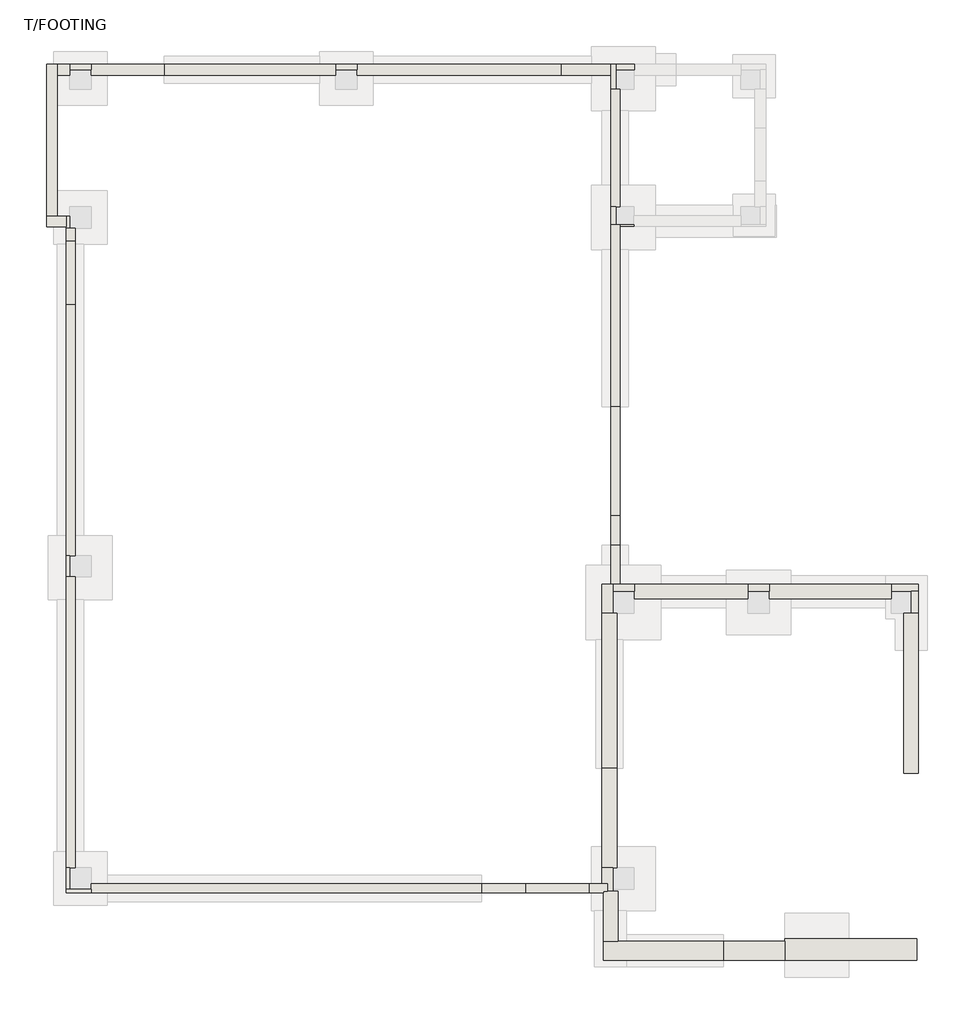
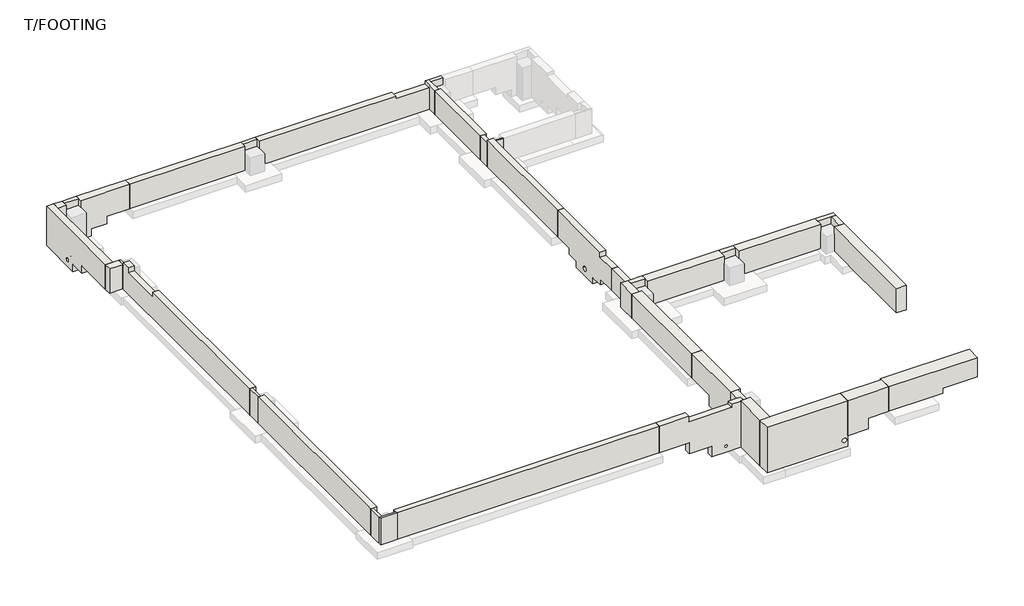
# One storey, part 1 of 3: 39 walls.
"""IFC4 building model written with IfcOpenShell, lengths in millimetres."""

from ifc_helpers import new_model, si_unit, point, frame, frame_2d, origin, place, context, project, spatial, polyline, circle_curve, trimmed, segment, composite_curve, outline, extrude, faceted_brep, element, save
from ifc_brep_helpers import plane_surface, revolved_surface, advanced_brep

model = new_model("IFC4")

# Units and contexts
model_context = context("Model", 3, world=origin())
ifc_project = project(units=[si_unit("LENGTHUNIT", "METRE", prefix="MILLI")], contexts=[model_context])

# Site, building, storey
site = spatial("IfcSite", under=ifc_project)
building = spatial("IfcBuilding", under=site)
storey = spatial("IfcBuildingStorey", under=building, Name="T/FOOTING", Elevation=-1092.2)

# Walls
placement = place(None, origin())
element("IfcWall", 1, ObjectType="10\" CONCRETE WALL", at=placement, inside=storey, context=model_context, shape_type="AdvancedBrep", body=[
    advanced_brep(
    [(-51687.4600821, -10190.4231529, -1092.2), (-52957.4600821, -10190.4231529, -1092.2), (-52957.4600821, -10190.4231529, 101.6), (-51700.1600824, -10190.4231529, 101.6), (-51700.1600824, -10190.4231529, -127.0), (-49871.3600824, -10190.4231529, -127.0), (-49871.3600824, -10190.4231529, 0.0), (-49512.5850821, -10190.4231529, 0.0), (-49360.1850821, -10190.4231529, 0.0), (-49360.1850821, -10190.4231529, -2057.4), (-49512.5850821, -10190.4231529, -2057.4), (-50722.2600821, -10190.4231529, -2057.4), (-50722.2600821, -10190.4231529, -1574.8), (-51687.4600821, -10190.4231529, -1574.8), (-50163.4600821, -10190.4231529, -1790.7), (-50061.8600821, -10190.4231529, -1790.7), (-52957.4600821, -10444.4231529, -1092.2), (-51687.4600821, -10444.4231529, -1092.2), (-51687.4600821, -10444.4231529, -1574.8), (-50722.2600821, -10444.4231529, -1574.8), (-50722.2600821, -10444.4231529, -2057.4), (-49477.6600821, -10444.4231529, -2057.4), (-49477.6600821, -10444.4231529, 0.0), (-49871.3600824, -10444.4231529, 0.0), (-49871.3600824, -10444.4231529, -127.0), (-51700.1600824, -10444.4231529, -127.0), (-51700.1600824, -10444.4231529, 101.6), (-52957.4600821, -10444.4231529, 101.6), (-50061.8600821, -10444.4231529, -1790.7), (-50163.4600821, -10444.4231529, -1790.7), (-49360.1850821, -10393.6231529, 0.0), (-49360.1850821, -10393.6231529, -2057.4), (-49477.6600821, -10393.6231529, -2057.4), (-49477.6600821, -10393.6231529, 0.0)],
    [
        (0, 1),
        (1, 2),
        (2, 3),
        (3, 4),
        (4, 5),
        (5, 6),
        (6, 7),
        (7, 8),
        (8, 9),
        (9, 10),
        (10, 11),
        (11, 12),
        (12, 13),
        (13, 0),
        (14, 15, circle_curve(frame((-50112.6600821, -10190.4231529, -1790.7), z_axis=(0.0, -1.0, 0.0), x_axis=(1.0, 0.0, 0.0)), 50.8)),
        (15, 14, circle_curve(frame((-50112.6600821, -10190.4231529, -1790.7), z_axis=(0.0, -1.0, 0.0), x_axis=(1.0, 0.0, 0.0)), 50.8)),
        (16, 17),
        (17, 18),
        (18, 19),
        (19, 20),
        (20, 21),
        (21, 22),
        (22, 23),
        (23, 24),
        (24, 25),
        (25, 26),
        (26, 27),
        (27, 16),
        (28, 29, circle_curve(frame((-50112.6600821, -10444.4231529, -1790.7), z_axis=(0.0, 1.0, 0.0), x_axis=(1.0, 0.0, 0.0)), 50.8)),
        (29, 28, circle_curve(frame((-50112.6600821, -10444.4231529, -1790.7), z_axis=(0.0, 1.0, 0.0), x_axis=(1.0, 0.0, 0.0)), 50.8)),
        (0, 17),
        (16, 1),
        (27, 2),
        (26, 3),
        (8, 30),
        (30, 31),
        (31, 9),
        (31, 32),
        (32, 21),
        (20, 11),
        (19, 12),
        (18, 13),
        (14, 29),
        (28, 15),
        (25, 4),
        (24, 5),
        (23, 6),
        (22, 33),
        (33, 30),
        (32, 33),
    ],
    [
        plane_surface(frame((-49360.1850821, -10190.4231529, -2057.4), z_axis=(0.0, 1.0, 0.0), x_axis=(-1.0, 0.0, 0.0))),
        plane_surface(frame((-49360.1850821, -10444.4231529, -2057.4), z_axis=(0.0, -1.0, 0.0), x_axis=(1.0, 0.0, 0.0))),
        plane_surface(frame((-51687.4600821, -10190.4231529, -1092.2), z_axis=(0.0, 0.0, -1.0), x_axis=(0.0, -1.0, 0.0))),
        plane_surface(frame((-52957.4600821, -10190.4231529, -1092.2), z_axis=(-1.0, 0.0, 0.0), x_axis=(0.0, -1.0, 0.0))),
        plane_surface(frame((-52957.4600821, -10190.4231529, 101.6), z_axis=(0.0, 0.0, 1.0), x_axis=(0.0, -1.0, 0.0))),
        plane_surface(frame((-49360.1850821, -10190.4231529, 0.0), z_axis=(1.0, 0.0, 0.0), x_axis=(0.0, -1.0, 0.0))),
        plane_surface(frame((-49360.1850821, -10190.4231529, -2057.4), z_axis=(0.0, 0.0, -1.0), x_axis=(0.0, -1.0, 0.0))),
        plane_surface(frame((-50722.2600821, -10190.4231529, -2057.4), z_axis=(-1.0, 0.0, 0.0), x_axis=(0.0, -1.0, 0.0))),
        plane_surface(frame((-50722.2600821, -10190.4231529, -1574.8), z_axis=(0.0, 0.0, -1.0), x_axis=(0.0, -1.0, 0.0))),
        plane_surface(frame((-51687.4600821, -10190.4231529, -1574.8), z_axis=(-1.0, 0.0, 0.0), x_axis=(0.0, -1.0, 0.0))),
        revolved_surface(polyline([(-50061.8600821, -10444.4231529, -1790.7), (-50061.8600821, -10190.4231529, -1790.7)]), (-50112.6600821, -10317.4231529, -1790.7), (0.0, -1.0, 0.0)),
        plane_surface(frame((-51700.1600824, -10190.4231529, 101.6), z_axis=(1.0, 0.0, 0.0), x_axis=(0.0, -1.0, 0.0))),
        plane_surface(frame((-51700.1600824, -10190.4231529, -127.0), z_axis=(0.0, 0.0, 1.0), x_axis=(0.0, -1.0, 0.0))),
        plane_surface(frame((-49871.3600824, -10190.4231529, -127.0), z_axis=(-1.0, 0.0, 0.0), x_axis=(0.0, -1.0, 0.0))),
        plane_surface(frame((-49871.3600824, -10190.4231529, 0.0), z_axis=(0.0, 0.0, 1.0), x_axis=(0.0, -1.0, 0.0))),
        plane_surface(frame((-49477.6600821, -12247.8231529, -2057.4), z_axis=(1.0, 0.0, 0.0), x_axis=(0.0, -1.0, 0.0))),
        plane_surface(frame((-49058.5600821, -10393.6231529, -2057.4), z_axis=(0.0, -1.0, 0.0), x_axis=(-1.0, 0.0, 0.0))),
    ],
    [
        (0, [[1, 2, 3, 4, 5, 6, 7, 8, 9, 10, 11, 12, 13, 14], [15, 16]]),
        (1, [[17, 18, 19, 20, 21, 22, 23, 24, 25, 26, 27, 28], [29, 30]]),
        (2, [[-1, 31, -17, 32]]),
        (3, [[-2, -32, -28, 33]]),
        (4, [[-3, -33, -27, 34]]),
        (5, [[-9, 35, 36, 37]]),
        (6, [[-11, -10, -37, 38, 39, -21, 40]]),
        (7, [[-12, -40, -20, 41]]),
        (8, [[-13, -41, -19, 42]]),
        (9, [[-14, -42, -18, -31]]),
        (10, [[-15, 43, -29, 44]]),
        (10, [[-16, -44, -30, -43]]),
        (11, [[-4, -34, -26, 45]]),
        (12, [[-5, -45, -25, 46]]),
        (13, [[-6, -46, -24, 47]]),
        (14, [[-8, -7, -47, -23, 48, 49, -35]]),
        (15, [[50, -48, -22, -39]]),
        (16, [[-50, -38, -36, -49]]),
    ],
),
])
element("IfcWall", 2, ObjectType="10\" CONCRETE WALL", at=placement, inside=storey, context=model_context, shape_type="Brep", body=[
    faceted_brep([(-64549.3850821, -9733.2231529, -1092.2), (-64549.3850821, -1436.1544032, -1092.2), (-64549.3850821, -1436.1544032, 101.6), (-64549.3850821, -9733.2231529, 101.6), (-64803.3850821, -9733.2231529, -1092.2), (-64803.3850821, -9733.2231529, 101.6), (-64803.3850821, -1436.1544032, 101.6), (-64803.3850821, -1436.1544032, -1092.2), (-64701.7850821, -9733.2231529, -1092.2), (-64701.7850821, -1436.1544032, -1092.2), (-64701.7850821, -1436.1544032, 101.6), (-64701.7850821, -9733.2231529, 101.6)], [[[0, 1, 2, 3]], [[4, 5, 6, 7]], [[1, 0, 8, 4, 7, 9]], [[2, 1, 9, 7, 6, 10]], [[3, 2, 10, 6, 5, 11]], [[0, 3, 11, 5, 4, 8]]]),
])
element("IfcWall", 3, ObjectType="10\" CONCRETE WALL", at=placement, inside=storey, context=model_context, shape_type="Brep", body=[
    faceted_brep([(-49007.7600821, 9117.3505048, -1092.2), (-49007.7600821, 12470.1505048, -1092.2), (-49007.7600821, 12470.1505048, 0.0), (-49007.7600821, 9117.3505048, 0.0), (-49261.7600821, 9117.3505048, -1092.2), (-49261.7600821, 9117.3505048, 0.0), (-49261.7600821, 12470.1505048, 0.0), (-49261.7600821, 12470.1505048, -1092.2), (-49109.3600821, 9117.3505048, -1092.2), (-49109.3600821, 12470.1505048, -1092.2), (-49109.3600821, 12470.1505048, 0.0), (-49109.3600821, 9117.3505048, 0.0)], [[[0, 1, 2, 3]], [[4, 5, 6, 7]], [[1, 0, 8, 4, 7, 9]], [[2, 1, 9, 7, 6, 10]], [[3, 2, 10, 6, 5, 11]], [[0, 3, 11, 5, 4, 8]]]),
])
element("IfcWall", 4, ObjectType="10\" CONCRETE WALL", at=placement, inside=storey, context=model_context, shape_type="Brep", body=[
    faceted_brep([(-49007.7600821, -1643.3231529, -1092.2), (-49007.7600821, -538.4231529, -1092.2), (-49007.7600821, -538.4231529, -127.0), (-49007.7600821, -1643.3231529, -127.0), (-49261.7600821, -1643.3231529, -1092.2), (-49261.7600821, -1643.3231529, -127.0), (-49261.7600821, -538.4231529, -127.0), (-49261.7600821, -538.4231529, -1092.2), (-49207.7850821, -1643.3231529, -1092.2)], [[[0, 1, 2, 3]], [[4, 5, 6, 7]], [[1, 0, 8, 4, 7]], [[2, 1, 7, 6]], [[3, 2, 6, 5]], [[0, 3, 5, 4, 8]]]),
])
element("IfcWall", 5, ObjectType="10\" CONCRETE WALL", at=placement, inside=storey, context=model_context, shape_type="Brep", body=[
    faceted_brep([(-64549.3850821, 8507.7505048, 101.6), (-64549.3850821, 8152.1505048, 101.6), (-64549.3850821, 8152.1505048, -127.0), (-64549.3850821, 6323.3505048, -127.0), (-64549.3850821, 6323.3505048, 101.6), (-64549.3850821, -826.5544032, 101.6), (-64549.3850821, -826.5544032, -1092.2), (-64549.3850821, 8507.7505048, -1092.2), (-64803.3850821, 8507.7505048, 101.6), (-64803.3850821, 8507.7505048, 0.0), (-64803.3850821, 8507.7505048, -1092.2), (-64803.3850821, -826.5544032, -1092.2), (-64803.3850821, -826.5544032, 101.6), (-64803.3850821, 6323.3505048, 101.6), (-64803.3850821, 6323.3505048, -127.0), (-64803.3850821, 8152.1505048, -127.0), (-64803.3850821, 8152.1505048, 101.6), (-64701.7850821, -826.5544032, -1092.2), (-64701.7850821, 8507.7505048, -1092.2), (-64701.7850821, -826.5544032, 101.6)], [[[0, 1, 2, 3, 4, 5, 6, 7]], [[8, 9, 10, 11, 12, 13, 14, 15, 16]], [[1, 0, 8, 16]], [[7, 6, 17, 11, 10, 18]], [[6, 5, 19, 12, 11, 17]], [[0, 7, 18, 10, 9, 8]], [[3, 2, 15, 14]], [[4, 3, 14, 13]], [[2, 1, 16, 15]], [[5, 4, 13, 12, 19]]]),
])
element("IfcWall", 6, ObjectType="10\" CONCRETE WALL", at=placement, inside=storey, context=model_context, shape_type="Brep", body=[
    faceted_brep([(-49007.7600821, 8609.3505048, 101.6), (-49007.7600821, 3423.9768471, 101.6), (-49007.7600821, 3423.9768471, -1092.2), (-49007.7600821, 8558.5505048, -1092.2), (-49007.7600821, 8609.3505048, -1092.2), (-49007.7600821, 8609.3505048, 0.0), (-49261.7600821, 8609.3505048, 101.6), (-49261.7600821, 8609.3505048, 0.0), (-49261.7600821, 8609.3505048, -1092.2), (-49261.7600821, 3423.9768471, -1092.2), (-49261.7600821, 3423.9768471, 101.6), (-49109.3600821, 8609.3505048, -1092.2)], [[[0, 1, 2, 3, 4, 5]], [[6, 7, 8, 9, 10]], [[1, 0, 6, 10]], [[4, 3, 2, 9, 8, 11]], [[2, 1, 10, 9]], [[0, 5, 4, 11, 8, 7, 6]]]),
])
element("IfcWall", 7, ObjectType="10\" CONCRETE WALL", at=placement, inside=storey, context=model_context, shape_type="SweptSolid", body=[
    extrude(outline(polyline([(325.1768471, 101.6), (3423.9768471, 101.6), (3423.9768471, -1092.2), (2585.7768471, -1092.2), (2585.7768471, -1358.9), (2052.3768471, -1358.9), (2052.3768471, -1625.6), (833.1768471, -1625.6), (833.1768471, -1358.9), (299.7768471, -1358.9), (299.7768471, -1092.2), (-538.4231529, -1092.2), (-538.4231529, -127.0), (325.1768471, -127.0), (325.1768471, 101.6)]), holes=[composite_curve([segment(trimmed(circle_curve(frame_2d((1442.7768471, -1320.8)), 101.6), [point((1544.3768471, -1320.8))], [point((1341.1768471, -1320.8))], True, "CARTESIAN"), True, "CONTINUOUS"), segment(trimmed(circle_curve(frame_2d((1442.7768471, -1320.8)), 101.6), [point((1341.1768471, -1320.8))], [point((1544.3768471, -1320.8))], True, "CARTESIAN"), True, "CONTINUOUS")], self_intersect=False)]), frame((-49261.7600821, 0.0, 0.0), z_axis=(1.0, 0.0, 0.0), x_axis=(0.0, 1.0, 0.0)), (0.0, 0.0, 1.0), 254.0),
])
element("IfcWall", 8, ObjectType="10\" CONCRETE WALL", at=placement, inside=storey, context=model_context, shape_type="Brep", body=[
    faceted_brep([(-52957.4600821, -10190.4231529, -1092.2), (-64092.1850821, -10190.4231529, -1092.2), (-64092.1850821, -10190.4231529, 101.6), (-52957.4600821, -10190.4231529, 101.6), (-52957.4600821, -10444.4231529, -1092.2), (-52957.4600821, -10444.4231529, 101.6), (-64092.1850821, -10444.4231529, 101.6), (-64092.1850821, -10444.4231529, -1092.2), (-64092.1850821, -10342.8231529, -1092.2), (-64092.1850821, -10342.8231529, 101.6)], [[[0, 1, 2, 3]], [[4, 5, 6, 7]], [[1, 0, 4, 7, 8]], [[2, 1, 8, 7, 6, 9]], [[3, 2, 9, 6, 5]], [[0, 3, 5, 4]]]),
])
element("IfcWall", 9, ObjectType="12\" CONCRETE WALL", at=placement, inside=storey, context=model_context, shape_type="AdvancedBrep", body=[
    advanced_brep(
    [(-65057.3850821, 8850.6505048, -1092.2), (-65057.3850821, 10577.8505048, -1092.2), (-65057.3850821, 10577.8505048, -1422.4), (-65057.3850821, 11238.2505048, -1422.4), (-65057.3850821, 11238.2505048, -1752.6), (-65057.3850821, 12876.5505048, -1752.6), (-65057.3850821, 13181.3505048, -1752.6), (-65057.3850821, 13181.3505048, 0.0), (-65057.3850821, 12876.5505048, 0.0), (-65057.3850821, 8850.6505048, 0.0), (-65057.3850821, 11720.8505048, -1460.5), (-65057.3850821, 11568.4505048, -1460.5), (-65362.1850821, 8850.6505048, -1092.2), (-65362.1850821, 8850.6505048, 0.0), (-65362.1850821, 13181.3505048, 0.0), (-65362.1850821, 13181.3505048, -1752.6), (-65362.1850821, 11238.2505048, -1752.6), (-65362.1850821, 11238.2505048, -1422.4), (-65362.1850821, 10577.8505048, -1422.4), (-65362.1850821, 10577.8505048, -1092.2), (-65362.1850821, 11720.8505048, -1460.5), (-65362.1850821, 11568.4505048, -1460.5)],
    [
        (0, 1),
        (1, 2),
        (2, 3),
        (3, 4),
        (4, 5),
        (5, 6),
        (6, 7),
        (7, 8),
        (8, 9),
        (9, 0),
        (10, 11, circle_curve(frame((-65057.3850821, 11644.6505048, -1460.5), z_axis=(-1.0, 0.0, 0.0), x_axis=(0.0, -1.0, 0.0)), 76.2)),
        (11, 10, circle_curve(frame((-65057.3850821, 11644.6505048, -1460.5), z_axis=(-1.0, 0.0, 0.0), x_axis=(0.0, -1.0, 0.0)), 76.2)),
        (12, 13),
        (13, 14),
        (14, 15),
        (15, 16),
        (16, 17),
        (17, 18),
        (18, 19),
        (19, 12),
        (20, 21, circle_curve(frame((-65362.1850821, 11644.6505048, -1460.5), z_axis=(1.0, 0.0, 0.0), x_axis=(0.0, -1.0, 0.0)), 76.2)),
        (21, 20, circle_curve(frame((-65362.1850821, 11644.6505048, -1460.5), z_axis=(1.0, 0.0, 0.0), x_axis=(0.0, -1.0, 0.0)), 76.2)),
        (6, 15),
        (14, 7),
        (9, 13),
        (12, 0),
        (19, 1),
        (18, 2),
        (17, 3),
        (16, 4),
        (10, 20),
        (21, 11),
    ],
    [
        plane_surface(frame((-65057.3850821, 8698.2505048, -1092.2), z_axis=(1.0, 0.0, 0.0), x_axis=(0.0, 1.0, 0.0))),
        plane_surface(frame((-65362.1850821, 8698.2505048, -1092.2), z_axis=(-1.0, 0.0, 0.0), x_axis=(0.0, -1.0, 0.0))),
        plane_surface(frame((-64657.3350821, 13181.3505048, -1752.6), z_axis=(0.0, 1.0, 0.0), x_axis=(-1.0, 0.0, 0.0))),
        plane_surface(frame((-64752.5850821, 8850.6505048, -1092.2), z_axis=(0.0, -1.0, 0.0), x_axis=(-1.0, 0.0, 0.0))),
        plane_surface(frame((-65057.3850821, 8698.2505048, -1092.2), z_axis=(0.0, 0.0, -1.0), x_axis=(-1.0, 0.0, 0.0))),
        plane_surface(frame((-65057.3850821, 13028.9505048, 0.0), z_axis=(0.0, 0.0, 1.0), x_axis=(-1.0, 0.0, 0.0))),
        plane_surface(frame((-65057.3850821, 10577.8505048, -1092.2), z_axis=(0.0, -1.0, 0.0), x_axis=(-1.0, 0.0, 0.0))),
        plane_surface(frame((-65057.3850821, 10577.8505048, -1422.4), z_axis=(0.0, 0.0, -1.0), x_axis=(-1.0, 0.0, 0.0))),
        plane_surface(frame((-65057.3850821, 11238.2505048, -1422.4), z_axis=(0.0, -1.0, 0.0), x_axis=(-1.0, 0.0, 0.0))),
        plane_surface(frame((-65057.3850821, 11238.2505048, -1752.6), z_axis=(0.0, 0.0, -1.0), x_axis=(-1.0, 0.0, 0.0))),
        revolved_surface(polyline([(-65362.1850821, 11568.4505048, -1460.5), (-65057.3850821, 11568.4505048, -1460.5)]), (-65209.7850821, 11644.6505048, -1460.5), (-1.0, 0.0, 0.0)),
    ],
    [
        (0, [[1, 2, 3, 4, 5, 6, 7, 8, 9, 10], [11, 12]]),
        (1, [[13, 14, 15, 16, 17, 18, 19, 20], [21, 22]]),
        (2, [[-7, 23, -15, 24]]),
        (3, [[-10, 25, -13, 26]]),
        (4, [[-1, -26, -20, 27]]),
        (5, [[-9, -8, -24, -14, -25]]),
        (6, [[-2, -27, -19, 28]]),
        (7, [[-3, -28, -18, 29]]),
        (8, [[-4, -29, -17, 30]]),
        (9, [[-6, -5, -30, -16, -23]]),
        (10, [[-11, 31, -22, 32]]),
        (10, [[-12, -32, -21, -31]]),
    ],
),
])
element("IfcWall", 10, ObjectType="12\" CONCRETE WALL", at=placement, inside=storey, context=model_context, shape_type="Brep", body=[
    faceted_brep([(-65057.3850821, 12876.5505048, -1752.6), (-64701.7850821, 12876.5505048, -1752.6), (-64701.7850821, 12876.5505048, 0.0), (-65057.3850821, 12876.5505048, 0.0), (-65057.3850821, 13181.3505048, -1752.6), (-65057.3850821, 13181.3505048, 0.0), (-64701.7850821, 13181.3505048, 0.0), (-64701.7850821, 13181.3505048, -1752.6), (-64701.7850821, 13028.9505048, -1752.6), (-64701.7850821, 13028.9505048, 0.0)], [[[0, 1, 2, 3]], [[4, 5, 6, 7]], [[1, 0, 4, 7, 8]], [[2, 1, 8, 7, 6, 9]], [[3, 2, 9, 6, 5]], [[0, 3, 5, 4]]]),
])
element("IfcWall", 11, ObjectType="12\" CONCRETE WALL", at=placement, inside=storey, context=model_context, shape_type="Brep", body=[
    faceted_brep([(-64803.3850821, 8850.6505048, -1092.2), (-65057.3850821, 8850.6505048, -1092.2), (-65362.1850821, 8850.6505048, -1092.2), (-65362.1850821, 8850.6505048, 0.0), (-65057.3850821, 8850.6505048, 0.0), (-64803.3850821, 8850.6505048, 0.0), (-64803.3850821, 8545.8505048, -1092.2), (-64803.3850821, 8545.8505048, 0.0), (-65362.1850821, 8545.8505048, 0.0), (-65362.1850821, 8545.8505048, -1092.2)], [[[0, 1, 2, 3, 4, 5]], [[6, 7, 8, 9]], [[3, 2, 9, 8]], [[2, 1, 0, 6, 9]], [[5, 4, 3, 8, 7]], [[0, 5, 7, 6]]]),
])
element("IfcWall", 12, ObjectType="12\" CONCRETE WALL", at=placement, inside=storey, context=model_context, shape_type="Brep", body=[
    faceted_brep([(-64092.1850821, 12876.5505048, -1752.6), (-63634.9850821, 12876.5505048, -1752.6), (-63634.9850821, 12876.5505048, -1422.4), (-62974.5850821, 12876.5505048, -1422.4), (-62974.5850821, 12876.5505048, -1092.2), (-62009.3850821, 12876.5505048, -1092.2), (-62009.3850821, 12876.5505048, 0.0), (-64092.1850821, 12876.5505048, 0.0), (-64092.1850821, 13181.3505048, -1752.6), (-64092.1850821, 13181.3505048, 0.0), (-62009.3850821, 13181.3505048, 0.0), (-62009.3850821, 13181.3505048, -1092.2), (-62974.5850821, 13181.3505048, -1092.2), (-62974.5850821, 13181.3505048, -1422.4), (-63634.9850821, 13181.3505048, -1422.4), (-63634.9850821, 13181.3505048, -1752.6), (-64092.1850821, 13028.9505048, -1752.6), (-64092.1850821, 13028.9505048, 0.0)], [[[0, 1, 2, 3, 4, 5, 6, 7]], [[8, 9, 10, 11, 12, 13, 14, 15]], [[1, 0, 16, 8, 15]], [[2, 1, 15, 14]], [[3, 2, 14, 13]], [[4, 3, 13, 12]], [[5, 4, 12, 11]], [[6, 5, 11, 10]], [[7, 6, 10, 9, 17]], [[0, 7, 17, 9, 8, 16]]]),
])
element("IfcWall", 13, ObjectType="12\" CONCRETE WALL", at=placement, inside=storey, context=model_context, shape_type="Brep", body=[
    faceted_brep([(-56500.7600821, 12876.5505048, -1092.2), (-49261.7600821, 12876.5505048, -1092.2), (-49261.7600821, 12876.5505048, -127.0), (-50684.1600821, 12876.5505048, -127.0), (-50684.1600821, 12876.5505048, 0.0), (-56500.7600821, 12876.5505048, 0.0), (-56500.7600821, 13181.3505048, -1092.2), (-56500.7600821, 13181.3505048, 0.0), (-50684.1600821, 13181.3505048, 0.0), (-50684.1600821, 13181.3505048, -127.0), (-49261.7600821, 13181.3505048, -127.0), (-49261.7600821, 13181.3505048, -1092.2), (-56500.7600821, 13028.9505048, -1092.2), (-56500.7600821, 13028.9505048, 0.0)], [[[0, 1, 2, 3, 4, 5]], [[6, 7, 8, 9, 10, 11]], [[2, 1, 11, 10]], [[1, 0, 12, 6, 11]], [[5, 4, 8, 7, 13]], [[0, 5, 13, 7, 6, 12]], [[3, 2, 10, 9]], [[4, 3, 9, 8]]]),
])
element("IfcWall", 14, ObjectType="12\" CONCRETE WALL", at=placement, inside=storey, context=model_context, shape_type="Brep", body=[
    faceted_brep([(-49512.5850821, -1643.3231529, 0.0), (-49512.5850821, -1643.3231529, -1092.2), (-49512.5850821, -2468.8231529, -1092.2), (-49512.5850821, -2468.8231529, 0.0), (-49207.7850821, -1643.3231529, -1092.2), (-49207.7850821, -1643.3231529, 0.0), (-49207.7850821, -1846.5231529, 0.0), (-49207.7850821, -2468.8231529, 0.0), (-49207.7850821, -2468.8231529, -304.8), (-49207.7850821, -2468.8231529, -1092.2), (-49207.7850821, -1859.2231529, -1092.2), (-49207.7850821, -1846.5231529, -1092.2), (-49261.7600821, -1643.3231529, -1092.2)], [[[0, 1, 2, 3]], [[4, 5, 6, 7, 8, 9, 10, 11]], [[2, 1, 12, 4, 11, 10, 9]], [[3, 2, 9, 8, 7]], [[0, 3, 7, 6, 5]], [[0, 5, 4, 12, 1]]]),
])
element("IfcWall", 15, ObjectType="12\" CONCRETE WALL", at=placement, inside=storey, context=model_context, shape_type="Brep", body=[
    faceted_brep([(-57110.3600821, 12876.5505048, 0.0), (-62009.3850821, 12876.5505048, 0.0), (-62009.3850821, 12876.5505048, -1092.2), (-57110.3600821, 12876.5505048, -1092.2), (-57110.3600821, 13181.3505048, 0.0), (-57110.3600821, 13181.3505048, -1092.2), (-62009.3850821, 13181.3505048, -1092.2), (-62009.3850821, 13181.3505048, 0.0), (-57110.3600821, 13028.9505048, 0.0), (-57110.3600821, 13028.9505048, -1092.2)], [[[0, 1, 2, 3]], [[4, 5, 6, 7]], [[1, 0, 8, 4, 7]], [[3, 2, 6, 5, 9]], [[2, 1, 7, 6]], [[0, 3, 9, 5, 4, 8]]]),
])
element("IfcWall", 16, ObjectType="12\" CONCRETE WALL", at=placement, inside=storey, context=model_context, shape_type="Brep", body=[
    faceted_brep([(-49207.7850821, -9733.2231529, 0.0), (-49207.7850821, -10393.6231529, 0.0), (-49207.7850821, -10393.6231529, -2057.4), (-49207.7850821, -10342.8231529, -2057.4), (-49207.7850821, -9733.2231529, -2057.4), (-49207.7850821, -9733.2231529, -304.8), (-49512.5850821, -9733.2231529, 0.0), (-49512.5850821, -9733.2231529, -2057.4), (-49512.5850821, -10190.4231529, -2057.4), (-49512.5850821, -10190.4231529, 0.0), (-49360.1850821, -10190.4231529, 0.0), (-49360.1850821, -10393.6231529, 0.0), (-49360.1850821, -10393.6231529, -2057.4), (-49360.1850821, -10190.4231529, -2057.4)], [[[0, 1, 2, 3, 4, 5]], [[6, 7, 8, 9]], [[1, 0, 6, 9, 10, 11]], [[2, 1, 11, 12]], [[4, 3, 2, 12, 13, 8, 7]], [[6, 0, 5, 4, 7]], [[13, 10, 9, 8]], [[10, 13, 12, 11]]]),
])
element("IfcWall", 17, ObjectType="16.5\" CONCRETE WALL", at=placement, inside=storey, context=model_context, shape_type="Brep", body=[
    faceted_brep([(-49058.5600821, -11827.1356529, -2057.4), (-49058.5600821, -10393.6231529, -2057.4), (-49058.5600821, -10393.6231529, 0.0), (-49058.5600821, -11827.1356529, 0.0), (-49477.6600821, -11827.1356529, -2057.4), (-49477.6600821, -11827.1356529, 0.0), (-49477.6600821, -10444.4231529, 0.0), (-49477.6600821, -10393.6231529, 0.0), (-49477.6600821, -10393.6231529, -2057.4), (-49477.6600821, -10444.4231529, -2057.4), (-49360.1850821, -10393.6231529, -2057.4), (-49207.7850821, -10393.6231529, -2057.4), (-49360.1850821, -10393.6231529, 0.0), (-49207.7850821, -10393.6231529, 0.0)], [[[0, 1, 2, 3]], [[4, 5, 6, 7, 8, 9]], [[1, 0, 4, 9, 8, 10, 11]], [[2, 1, 11, 10, 8, 7, 12, 13]], [[3, 2, 13, 12, 7, 6, 5]], [[0, 3, 5, 4]]]),
])
element("IfcWall", 18, ObjectType="16.5\" CONCRETE WALL", at=placement, inside=storey, context=model_context, shape_type="Brep", body=[
    faceted_brep([(-40901.9850821, -2468.8231529, -1092.2), (-40901.9850821, -7036.0606529, -1092.2), (-40901.9850821, -7036.0606529, 0.0), (-40901.9850821, -2468.8231529, 0.0), (-40482.8850821, -2468.8231529, -1092.2), (-40482.8850821, -2468.8231529, 0.0), (-40482.8850821, -4348.4231529, 0.0), (-40482.8850821, -4602.4231529, 0.0), (-40482.8850821, -7036.0606529, 0.0), (-40482.8850821, -7036.0606529, -1092.2), (-40686.0850821, -2468.8231529, -1092.2), (-40686.0850821, -2468.8231529, 0.0)], [[[0, 1, 2, 3]], [[4, 5, 6, 7, 8, 9]], [[1, 0, 10, 4, 9]], [[2, 1, 9, 8]], [[3, 2, 8, 7, 6, 5, 11]], [[0, 3, 11, 5, 4, 10]]]),
])
element("IfcWall", 19, ObjectType="16.5\" CONCRETE WALL", at=placement, inside=storey, context=model_context, shape_type="Brep", body=[
    faceted_brep([(-49093.4850821, -9733.2231529, -2057.4), (-49093.4850821, -9123.6231529, -2057.4), (-49093.4850821, -9123.6231529, -1574.8), (-49093.4850821, -8158.4231529, -1574.8), (-49093.4850821, -8158.4231529, -1092.2), (-49093.4850821, -6888.4231529, -1092.2), (-49093.4850821, -6888.4231529, 0.0), (-49093.4850821, -9733.2231529, 0.0), (-49512.5850821, -9733.2231529, -2057.4), (-49512.5850821, -9733.2231529, 0.0), (-49512.5850821, -6888.4231529, 0.0), (-49512.5850821, -6888.4231529, -1092.2), (-49512.5850821, -8158.4231529, -1092.2), (-49512.5850821, -8158.4231529, -1574.8), (-49512.5850821, -9123.6231529, -1574.8), (-49512.5850821, -9123.6231529, -2057.4), (-49207.7850821, -9733.2231529, 0.0), (-49207.7850821, -9733.2231529, -2057.4)], [[[0, 1, 2, 3, 4, 5, 6, 7]], [[8, 9, 10, 11, 12, 13, 14, 15]], [[5, 4, 12, 11]], [[6, 5, 11, 10]], [[7, 6, 10, 9, 16]], [[0, 7, 16, 9, 8, 17]], [[1, 0, 17, 8, 15]], [[2, 1, 15, 14]], [[3, 2, 14, 13]], [[4, 3, 13, 12]]]),
])
element("IfcWall", 20, ObjectType="16.5\" CONCRETE WALL", at=placement, inside=storey, context=model_context, shape_type="Brep", body=[
    faceted_brep([(-44741.4490821, -2062.4231529, -1092.2), (-41257.5850821, -2062.4231529, -1092.2), (-41257.5850821, -2062.4231529, 0.0), (-44741.4490821, -2062.4231529, 0.0), (-44741.4490821, -1643.3231529, -1092.2), (-44741.4490821, -1643.3231529, 0.0), (-41257.5850821, -1643.3231529, 0.0), (-41257.5850821, -1643.3231529, -1092.2), (-44741.4490821, -1859.2231529, -1092.2), (-44741.4490821, -1846.5231529, -1092.2), (-41257.5850821, -1846.5231529, -1092.2), (-41257.5850821, -1859.2231529, -1092.2), (-41257.5850821, -1846.5231529, 0.0), (-44741.4490821, -1846.5231529, 0.0)], [[[0, 1, 2, 3]], [[4, 5, 6, 7]], [[1, 0, 8, 9, 4, 7, 10, 11]], [[2, 1, 11, 10, 7, 6, 12]], [[3, 2, 12, 6, 5, 13]], [[0, 3, 13, 5, 4, 9, 8]]]),
])
element("IfcWall", 21, ObjectType="16.5\" CONCRETE WALL", at=placement, inside=storey, context=model_context, shape_type="Brep", body=[
    faceted_brep([(-48595.0100821, -2062.4231529, -1092.2), (-45351.0490821, -2062.4231529, -1092.2), (-45351.0490821, -2062.4231529, 0.0), (-48595.0100821, -2062.4231529, 0.0), (-48595.0100821, -1643.3231529, -1092.2), (-48595.0100821, -1643.3231529, 0.0), (-45351.0490821, -1643.3231529, 0.0), (-45351.0490821, -1643.3231529, -1092.2), (-48595.0100821, -1846.5231529, -1092.2), (-45351.0490821, -1846.5231529, -1092.2), (-45351.0490821, -1859.2231529, -1092.2), (-45351.0490821, -1846.5231529, 0.0), (-48595.0100821, -1846.5231529, 0.0)], [[[0, 1, 2, 3]], [[4, 5, 6, 7]], [[1, 0, 8, 4, 7, 9, 10]], [[2, 1, 10, 9, 7, 6, 11]], [[3, 2, 11, 6, 5, 12]], [[0, 3, 12, 5, 4, 8]]]),
])
element("IfcWall", 22, ObjectType="16.5\" CONCRETE WALL", at=placement, inside=storey, context=model_context, shape_type="Brep", body=[
    faceted_brep([(-49093.4850821, -6888.4231529, -1092.2), (-49093.4850821, -2468.8231529, -1092.2), (-49093.4850821, -2468.8231529, 0.0), (-49093.4850821, -6888.4231529, 0.0), (-49512.5850821, -6888.4231529, -1092.2), (-49512.5850821, -6888.4231529, 0.0), (-49512.5850821, -2468.8231529, 0.0), (-49512.5850821, -2468.8231529, -1092.2), (-49207.7850821, -2468.8231529, -1092.2), (-49207.7850821, -2468.8231529, 0.0)], [[[0, 1, 2, 3]], [[4, 5, 6, 7]], [[1, 0, 4, 7, 8]], [[2, 1, 8, 7, 6, 9]], [[3, 2, 9, 6, 5]], [[0, 3, 5, 4]]]),
])
element("IfcWall", 23, ObjectType="2\" CONCRETE WALL", at=placement, inside=storey, context=model_context, shape_type="Brep", body=[
    faceted_brep([(-49007.7600821, 8558.5505048, -1092.2), (-48601.3600821, 8558.5505048, -1092.2), (-48601.3600821, 8558.5505048, 0.0), (-49007.7600821, 8558.5505048, 0.0), (-49007.7600821, 8609.3505048, -1092.2), (-49007.7600821, 8609.3505048, 0.0), (-48601.3600821, 8609.3505048, 0.0), (-48601.3600821, 8609.3505048, -304.8), (-48601.3600821, 8609.3505048, -1092.2)], [[[0, 1, 2, 3]], [[4, 5, 6, 7, 8]], [[1, 0, 4, 8]], [[2, 1, 8, 7, 6]], [[3, 2, 6, 5]], [[0, 3, 5, 4]]]),
])
element("IfcWall", 24, ObjectType="21\" CONCRETE WALL", at=placement, inside=storey, context=model_context, shape_type="SweptSolid", body=[
    extrude(outline(polyline([(-1092.2, -44302.2909443), (0.0, -44302.2909443), (0.0, -46055.0100821), (-1574.8, -46055.0100821), (-1574.8, -45178.5909443), (-1092.2, -45178.5909443), (-1092.2, -44302.2909443)])), frame((0.0, -12360.5356529, 0.0), z_axis=(0.0, 1.0, 0.0), x_axis=(0.0, 0.0, 1.0)), (0.0, 0.0, 1.0), 533.4),
])
element("IfcWall", 25, ObjectType="21\" CONCRETE WALL", at=placement, inside=storey, context=model_context, shape_type="AdvancedBrep", body=[
    advanced_brep(
    [(-46055.0100821, -11827.1356529, 0.0), (-46055.0100821, -11827.1356529, -1574.8), (-46055.0100821, -11827.1356529, -2057.4), (-49058.5600821, -11827.1356529, -2057.4), (-49477.6600821, -11827.1356529, -2057.4), (-49477.6600821, -11827.1356529, 0.0), (-49058.5600821, -11827.1356529, 0.0), (-46289.9600821, -11827.1356529, -1739.9), (-46086.7600821, -11827.1356529, -1739.9), (-46055.0100821, -12360.5356529, -2057.4), (-46055.0100821, -12360.5356529, -1574.8), (-46055.0100821, -12360.5356529, 0.0), (-49477.6600821, -12360.5356529, 0.0), (-49477.6600821, -12360.5356529, -2057.4), (-46289.9600821, -12360.5356529, -1739.9), (-46086.7600821, -12360.5356529, -1739.9)],
    [
        (0, 1),
        (1, 2),
        (2, 3),
        (3, 4),
        (4, 5),
        (5, 6),
        (6, 0),
        (7, 8, circle_curve(frame((-46188.3600821, -11827.1356529, -1739.9), z_axis=(0.0, -1.0, 0.0), x_axis=(1.0, 0.0, 0.0)), 101.6)),
        (8, 7, circle_curve(frame((-46188.3600821, -11827.1356529, -1739.9), z_axis=(0.0, -1.0, 0.0), x_axis=(1.0, 0.0, 0.0)), 101.6)),
        (9, 10),
        (10, 11),
        (11, 12),
        (12, 13),
        (13, 9),
        (14, 15, circle_curve(frame((-46188.3600821, -12360.5356529, -1739.9), z_axis=(0.0, 1.0, 0.0), x_axis=(1.0, 0.0, 0.0)), 101.6)),
        (15, 14, circle_curve(frame((-46188.3600821, -12360.5356529, -1739.9), z_axis=(0.0, 1.0, 0.0), x_axis=(1.0, 0.0, 0.0)), 101.6)),
        (4, 13),
        (12, 5),
        (2, 9),
        (11, 0),
        (7, 14),
        (15, 8),
    ],
    [
        plane_surface(frame((-46055.0100821, -11827.1356529, -2057.4), z_axis=(0.0, 1.0, 0.0), x_axis=(-1.0, 0.0, 0.0))),
        plane_surface(frame((-46055.0100821, -12360.5356529, -2057.4), z_axis=(0.0, -1.0, 0.0), x_axis=(1.0, 0.0, 0.0))),
        plane_surface(frame((-49477.6600821, -12247.8231529, -2057.4), z_axis=(-1.0, 0.0, 0.0), x_axis=(0.0, -1.0, 0.0))),
        plane_surface(frame((-46055.0100821, -11827.1356529, -2057.4), z_axis=(0.0, 0.0, -1.0), x_axis=(0.0, -1.0, 0.0))),
        plane_surface(frame((-49268.1100821, -11827.1356529, 0.0), z_axis=(0.0, 0.0, 1.0), x_axis=(0.0, -1.0, 0.0))),
        plane_surface(frame((-46055.0100821, -11827.1356529, 0.0), z_axis=(1.0, 0.0, 0.0), x_axis=(0.0, -1.0, 0.0))),
        revolved_surface(polyline([(-46086.7600821, -12360.5356529, -1739.9), (-46086.7600821, -11827.1356529, -1739.9)]), (-46188.3600821, -12093.8356529, -1739.9), (0.0, -1.0, 0.0)),
    ],
    [
        (0, [[1, 2, 3, 4, 5, 6, 7], [8, 9]]),
        (1, [[10, 11, 12, 13, 14], [15, 16]]),
        (2, [[-5, 17, -13, 18]]),
        (3, [[-4, -3, 19, -14, -17]]),
        (4, [[-7, -6, -18, -12, 20]]),
        (5, [[-20, -11, -10, -19, -2, -1]]),
        (6, [[-8, 21, -16, 22]]),
        (6, [[-9, -22, -15, -21]]),
    ],
),
])
element("IfcWall", 26, ObjectType="24\" CONCRETE WALL", at=placement, inside=storey, context=model_context, shape_type="Brep", body=[
    faceted_brep([(-40530.3909443, -11750.9356529, -863.6), (-42003.5909443, -11750.9356529, -863.6), (-42003.5909443, -11750.9356529, -1092.2), (-44302.2909443, -11750.9356529, -1092.2), (-44302.2909443, -11750.9356529, 0.0), (-40530.3909443, -11750.9356529, 0.0), (-40530.3909443, -12360.5356529, -863.6), (-40530.3909443, -12360.5356529, 0.0), (-44302.2909443, -12360.5356529, 0.0), (-44302.2909443, -12360.5356529, -1092.2), (-42003.5909443, -12360.5356529, -1092.2), (-42003.5909443, -12360.5356529, -863.6), (-44302.2909443, -11827.1356529, -1092.2), (-44302.2909443, -11827.1356529, 0.0)], [[[0, 1, 2, 3, 4, 5]], [[6, 7, 8, 9, 10, 11]], [[3, 2, 10, 9, 12]], [[4, 3, 12, 9, 8, 13]], [[5, 4, 13, 8, 7]], [[0, 5, 7, 6]], [[1, 0, 6, 11]], [[2, 1, 11, 10]]]),
])
element("IfcWall", 27, ObjectType="4\" CONCRETE WALL", at=placement, inside=storey, context=model_context, shape_type="Brep", body=[
    faceted_brep([(-64092.1850821, -10342.8231529, -1092.2), (-64701.7850821, -10342.8231529, -1092.2), (-64803.3850821, -10342.8231529, -1092.2), (-64803.3850821, -10342.8231529, 101.6), (-64701.7850821, -10342.8231529, 101.6), (-64092.1850821, -10342.8231529, 101.6), (-64092.1850821, -10342.8231529, -304.8), (-64092.1850821, -10444.4231529, -1092.2), (-64092.1850821, -10444.4231529, 101.6), (-64803.3850821, -10444.4231529, 101.6), (-64803.3850821, -10444.4231529, -1092.2)], [[[0, 1, 2, 3, 4, 5, 6]], [[7, 8, 9, 10]], [[2, 1, 0, 7, 10]], [[5, 4, 3, 9, 8]], [[0, 6, 5, 8, 7]], [[3, 2, 10, 9]]]),
])
element("IfcWall", 28, ObjectType="4\" CONCRETE WALL", at=placement, inside=storey, context=model_context, shape_type="Brep", body=[
    faceted_brep([(-64701.7850821, -10342.8231529, -1092.2), (-64701.7850821, -9733.2231529, -1092.2), (-64701.7850821, -9733.2231529, -304.8), (-64701.7850821, -9733.2231529, 101.6), (-64701.7850821, -10342.8231529, 101.6), (-64701.7850821, -10342.8231529, -304.8), (-64803.3850821, -10342.8231529, -1092.2), (-64803.3850821, -10342.8231529, 101.6), (-64803.3850821, -9733.2231529, 101.6), (-64803.3850821, -9733.2231529, -1092.2)], [[[0, 1, 2, 3, 4, 5]], [[6, 7, 8, 9]], [[1, 0, 6, 9]], [[3, 2, 1, 9, 8]], [[4, 3, 8, 7]], [[0, 5, 4, 7, 6]]]),
])
element("IfcWall", 29, ObjectType="4\" CONCRETE WALL", at=placement, inside=storey, context=model_context, shape_type="Brep", body=[
    faceted_brep([(-64701.7850821, -1436.1544032, -1092.2), (-64701.7850821, -826.5544032, -1092.2), (-64701.7850821, -826.5544032, -304.8), (-64701.7850821, -826.5544032, 101.6), (-64701.7850821, -1436.1544032, 101.6), (-64701.7850821, -1436.1544032, -304.8), (-64803.3850821, -1436.1544032, -1092.2), (-64803.3850821, -1436.1544032, 101.6), (-64803.3850821, -826.5544032, 101.6), (-64803.3850821, -826.5544032, -1092.2)], [[[0, 1, 2, 3, 4, 5]], [[6, 7, 8, 9]], [[1, 0, 6, 9]], [[3, 2, 1, 9, 8]], [[4, 3, 8, 7]], [[0, 5, 4, 7, 6]]]),
])
element("IfcWall", 30, ObjectType="4\" CONCRETE WALL", at=placement, inside=storey, context=model_context, shape_type="Brep", body=[
    faceted_brep([(-64701.7850821, 8850.6505048, 0.0), (-64701.7850821, 8507.7505048, 0.0), (-64701.7850821, 8507.7505048, -304.8), (-64701.7850821, 8507.7505048, -1092.2), (-64701.7850821, 8850.6505048, -1092.2), (-64803.3850821, 8850.6505048, 0.0), (-64803.3850821, 8850.6505048, -1092.2), (-64803.3850821, 8545.8505048, -1092.2), (-64803.3850821, 8507.7505048, -1092.2), (-64803.3850821, 8507.7505048, 0.0), (-64803.3850821, 8545.8505048, 0.0)], [[[0, 1, 2, 3, 4]], [[5, 6, 7, 8, 9, 10]], [[1, 0, 5, 10, 9]], [[4, 3, 8, 7, 6]], [[3, 2, 1, 9, 8]], [[0, 4, 6, 5]]]),
])
element("IfcWall", 31, ObjectType="6\" CONCRETE WALL", at=placement, inside=storey, context=model_context, shape_type="Brep", body=[
    faceted_brep([(-64701.7850821, 13028.9505048, -1752.6), (-64092.1850821, 13028.9505048, -1752.6), (-64092.1850821, 13028.9505048, -304.8), (-64092.1850821, 13028.9505048, 0.0), (-64701.7850821, 13028.9505048, 0.0), (-64701.7850821, 13028.9505048, -304.8), (-64701.7850821, 13181.3505048, -1752.6), (-64701.7850821, 13181.3505048, 0.0), (-64092.1850821, 13181.3505048, 0.0), (-64092.1850821, 13181.3505048, -1752.6)], [[[0, 1, 2, 3, 4, 5]], [[6, 7, 8, 9]], [[1, 0, 6, 9]], [[4, 3, 8, 7]], [[0, 5, 4, 7, 6]], [[1, 9, 8, 3, 2]]]),
])
element("IfcWall", 32, ObjectType="6\" CONCRETE WALL", at=placement, inside=storey, context=model_context, shape_type="Brep", body=[
    faceted_brep([(-57110.3600821, 13028.9505048, -1092.2), (-56500.7600821, 13028.9505048, -1092.2), (-56500.7600821, 13028.9505048, -304.8), (-56500.7600821, 13028.9505048, 0.0), (-57110.3600821, 13028.9505048, 0.0), (-57110.3600821, 13028.9505048, -304.8), (-57110.3600821, 13181.3505048, -1092.2), (-57110.3600821, 13181.3505048, 0.0), (-56500.7600821, 13181.3505048, 0.0), (-56500.7600821, 13181.3505048, -1092.2)], [[[0, 1, 2, 3, 4, 5]], [[6, 7, 8, 9]], [[1, 0, 6, 9]], [[3, 2, 1, 9, 8]], [[4, 3, 8, 7]], [[0, 5, 4, 7, 6]]]),
])
element("IfcWall", 33, ObjectType="6\" CONCRETE WALL", at=placement, inside=storey, context=model_context, shape_type="Brep", body=[
    faceted_brep([(-49109.3600821, 13028.9505048, 0.0), (-49109.3600821, 13028.9505048, -304.8), (-49109.3600821, 13028.9505048, -1092.2), (-48601.3600821, 13028.9505048, -1092.2), (-48595.0100821, 13028.9505048, -1092.2), (-48595.0100821, 13028.9505048, 0.0), (-49109.3600821, 13181.3505048, -1092.2), (-49109.3600821, 13181.3505048, 0.0), (-48595.0100821, 13181.3505048, 0.0), (-48595.0100821, 13181.3505048, -1092.2)], [[[0, 1, 2, 3, 4, 5]], [[6, 7, 8, 9]], [[4, 3, 2, 6, 9]], [[5, 4, 9, 8]], [[0, 5, 8, 7]], [[0, 7, 6, 2, 1]]]),
])
element("IfcWall", 34, ObjectType="6\" CONCRETE WALL", at=placement, inside=storey, context=model_context, shape_type="Brep", body=[
    faceted_brep([(-49109.3600821, 8609.3505048, -1092.2), (-49109.3600821, 9117.3505048, -1092.2), (-49109.3600821, 9117.3505048, -304.8), (-49109.3600821, 9117.3505048, 0.0), (-49109.3600821, 8609.3505048, 0.0), (-49109.3600821, 8609.3505048, -304.8), (-49261.7600821, 8609.3505048, -1092.2), (-49261.7600821, 8609.3505048, 0.0), (-49261.7600821, 9117.3505048, 0.0), (-49261.7600821, 9117.3505048, -1092.2)], [[[0, 1, 2, 3, 4, 5]], [[6, 7, 8, 9]], [[1, 0, 6, 9]], [[3, 2, 1, 9, 8]], [[4, 3, 8, 7]], [[0, 5, 4, 7, 6]]]),
])
element("IfcWall", 35, ObjectType="6\" CONCRETE WALL", at=placement, inside=storey, context=model_context, shape_type="Brep", body=[
    faceted_brep([(-49109.3600821, 12470.1505048, -1092.2), (-49109.3600821, 13028.9505048, -1092.2), (-49109.3600821, 13181.3505048, -1092.2), (-49109.3600821, 13181.3505048, 0.0), (-49109.3600821, 13028.9505048, 0.0), (-49109.3600821, 12470.1505048, 0.0), (-49109.3600821, 12470.1505048, -304.8), (-49261.7600821, 12470.1505048, -1092.2), (-49261.7600821, 12470.1505048, 0.0), (-49261.7600821, 13181.3505048, 0.0), (-49261.7600821, 13181.3505048, -127.0), (-49261.7600821, 13181.3505048, -1092.2), (-49261.7600821, 12876.5505048, -1092.2)], [[[0, 1, 2, 3, 4, 5, 6]], [[7, 8, 9, 10, 11, 12]], [[2, 1, 0, 7, 12, 11]], [[5, 4, 3, 9, 8]], [[0, 6, 5, 8, 7]], [[3, 2, 11, 10, 9]]]),
])
element("IfcWall", 36, ObjectType="8\" CONCRETE WALL", at=placement, inside=storey, context=model_context, shape_type="Brep", body=[
    faceted_brep([(-41257.5850821, -1846.5231529, -1092.2), (-40686.0850821, -1846.5231529, -1092.2), (-40482.8850821, -1846.5231529, -1092.2), (-40482.8850821, -1846.5231529, 0.0), (-40686.0850821, -1846.5231529, 0.0), (-41257.5850821, -1846.5231529, 0.0), (-41257.5850821, -1643.3231529, -1092.2), (-41257.5850821, -1643.3231529, 0.0), (-40482.8850821, -1643.3231529, 0.0), (-40482.8850821, -1643.3231529, -1092.2)], [[[0, 1, 2, 3, 4, 5]], [[6, 7, 8, 9]], [[2, 1, 0, 6, 9]], [[5, 4, 3, 8, 7]], [[0, 5, 7, 6]], [[3, 2, 9, 8]]]),
])
element("IfcWall", 37, ObjectType="8\" CONCRETE WALL", at=placement, inside=storey, context=model_context, shape_type="Brep", body=[
    faceted_brep([(-40686.0850821, -1846.5231529, -1092.2), (-40686.0850821, -1859.2231529, -1092.2), (-40686.0850821, -2468.8231529, -1092.2), (-40686.0850821, -2468.8231529, -304.8), (-40686.0850821, -2468.8231529, 0.0), (-40686.0850821, -1846.5231529, 0.0), (-40482.8850821, -1846.5231529, -1092.2), (-40482.8850821, -1846.5231529, 0.0), (-40482.8850821, -2468.8231529, 0.0), (-40482.8850821, -2468.8231529, -1092.2)], [[[0, 1, 2, 3, 4, 5]], [[6, 7, 8, 9]], [[2, 1, 0, 6, 9]], [[4, 3, 2, 9, 8]], [[5, 4, 8, 7]], [[0, 5, 7, 6]]]),
])
element("IfcWall", 38, ObjectType="8\" CONCRETE WALL", at=placement, inside=storey, context=model_context, shape_type="SweptSolid", body=[
    extrude(outline(polyline([(-44741.4490821, -1846.5231529), (-45351.0490821, -1846.5231529), (-45351.0490821, -1643.3231529), (-44741.4490821, -1643.3231529), (-44741.4490821, -1846.5231529)])), frame((0.0, 0.0, -1092.2), z_axis=(0.0, 0.0, 1.0), x_axis=(1.0, 0.0, 0.0)), (0.0, 0.0, 1.0), 1092.2),
])
element("IfcWall", 39, ObjectType="8\" CONCRETE WALL", at=placement, inside=storey, context=model_context, shape_type="Brep", body=[
    faceted_brep([(-49207.7850821, -1846.5231529, 0.0), (-49207.7850821, -1846.5231529, -1092.2), (-48595.0100821, -1846.5231529, -1092.2), (-48595.0100821, -1846.5231529, 0.0), (-49207.7850821, -1643.3231529, -1092.2), (-49207.7850821, -1643.3231529, 0.0), (-48595.0100821, -1643.3231529, 0.0), (-48595.0100821, -1643.3231529, -1092.2), (-49007.7600821, -1643.3231529, -1092.2)], [[[0, 1, 2, 3]], [[4, 5, 6, 7, 8]], [[2, 1, 4, 8, 7]], [[3, 2, 7, 6]], [[0, 3, 6, 5]], [[0, 5, 4, 1]]]),
])

save(model, "model.ifc")

# Revit data of these elements
# Type "10\" CONCRETE WALL"
#   Assembly Code = "B2010158"
#   Layers, outside or top first: 0' - 10" "Concrete, Cast-in-Place gray" (function 1)
# Type "12\" CONCRETE WALL"
#   Assembly Code = "B2010158"
#   Layers, outside or top first: 1' - 0" "Concrete, Cast-in-Place gray" (function 1)
# Type "16.5\" CONCRETE WALL"
#   Assembly Code = "B2010158"
#   Layers, outside or top first: 1' - 4 1/2" "Concrete, Cast-in-Place gray" (function 1)
# Type "2\" CONCRETE WALL"
#   Assembly Code = "B2010158"
#   Layers, outside or top first: 0' - 2" "Concrete, Cast-in-Place gray" (function 1)
# Type "21\" CONCRETE WALL"
#   Assembly Code = "B2010158"
#   Layers, outside or top first: 1' - 9" "Concrete, Cast-in-Place gray" (function 1)
# Type "24\" CONCRETE WALL"
#   Assembly Code = "B2010158"
#   Layers, outside or top first: 2' - 0" "Concrete, Cast-in-Place gray" (function 1)
# Type "4\" CONCRETE WALL"
#   Assembly Code = "B2010158"
#   Layers, outside or top first: 0' - 4" "Concrete, Cast-in-Place gray" (function 1)
# Type "6\" CONCRETE WALL"
#   Assembly Code = "B2010158"
#   Layers, outside or top first: 0' - 6" "Concrete, Cast-in-Place gray" (function 1)
# Type "8\" CONCRETE WALL"
#   Assembly Code = "B2010158"
#   Layers, outside or top first: 0' - 8" "Concrete, Cast-in-Place gray" (function 1)
# Elements 1, 2, 5, 6, 7, 8 (IfcWall, "10\" CONCRETE WALL")
#   Comments = ""
#   Top Offset = 0' - 4"
#   Base Offset = 0' - 0"
#   wall height = 3' - 11"
#   Phase Created = New Construction
#   Base Constraint = T/FOOTING
#   Top Constraint = MAIN LEVEL FLOOR PLAN
#   Materials on its faces: "Concrete, Cast-in-Place gray"
# Element 3 (IfcWall, "10\" CONCRETE WALL")
#   Comments = ""
#   Top Offset = 0' - 0"
#   Base Offset = 0' - 0"
#   wall height = 3' - 7"
#   Phase Created = New Construction
#   Base Constraint = T/FOOTING
#   Top Constraint = MAIN LEVEL FLOOR PLAN
#   Materials on its faces: "Concrete, Cast-in-Place gray"
# Element 4 (IfcWall, "10\" CONCRETE WALL")
#   Comments = ""
#   Top Offset = -0' - 5"
#   Base Offset = 0' - 0"
#   wall height = 3' - 2"
#   Phase Created = New Construction
#   Base Constraint = T/FOOTING
#   Top Constraint = MAIN LEVEL FLOOR PLAN
#   Materials on its faces: "Concrete, Cast-in-Place gray"
# Elements 9, 11, 12, 13, 14, 15, 16 (IfcWall, "12\" CONCRETE WALL")
#   Comments = ""
#   Top Offset = 0' - 0"
#   Base Offset = 0' - 0"
#   wall height = 3' - 7"
#   Phase Created = New Construction
#   Base Constraint = T/FOOTING
#   Top Constraint = MAIN LEVEL FLOOR PLAN
#   Materials on its faces: "Concrete, Cast-in-Place gray"
# Element 10 (IfcWall, "12\" CONCRETE WALL")
#   Comments = ""
#   built-in parameter 1001111 = -2' - 2"
#   Top Offset = 0' - 0"
#   Base Offset = -2' - 2"
#   wall height = 5' - 9"
#   Phase Created = New Construction
#   Base Constraint = T/FOOTING
#   Top Constraint = MAIN LEVEL FLOOR PLAN
#   Materials on its faces: "Concrete, Cast-in-Place gray"
# Element 17 (IfcWall, "16.5\" CONCRETE WALL")
#   Comments = ""
#   built-in parameter 1001111 = -3' - 2"
#   Top Offset = 0' - 0"
#   Base Offset = -3' - 2"
#   wall height = 6' - 9"
#   Phase Created = New Construction
#   Base Constraint = T/FOOTING
#   Top Constraint = MAIN LEVEL FLOOR PLAN
#   Materials on its faces: "Concrete, Cast-in-Place gray"
# Elements 18, 19, 20, 21, 22 (IfcWall, "16.5\" CONCRETE WALL")
#   Comments = ""
#   Top Offset = 0' - 0"
#   Base Offset = 0' - 0"
#   wall height = 3' - 7"
#   Phase Created = New Construction
#   Base Constraint = T/FOOTING
#   Top Constraint = MAIN LEVEL FLOOR PLAN
#   Materials on its faces: "Concrete, Cast-in-Place gray"
# Element 23 (IfcWall, "2\" CONCRETE WALL")
#   Comments = ""
#   Top Offset = 0' - 0"
#   Base Offset = 0' - 0"
#   wall height = 3' - 7"
#   Phase Created = New Construction
#   Base Constraint = T/FOOTING
#   Top Constraint = MAIN LEVEL FLOOR PLAN
#   Materials on its faces: "Concrete, Cast-in-Place gray"
# Element 24 (IfcWall, "21\" CONCRETE WALL")
#   Comments = ""
#   Top Offset = 0' - 0"
#   Base Offset = 0' - 0"
#   wall height = 3' - 7"
#   Phase Created = New Construction
#   Base Constraint = T/FOOTING
#   Top Constraint = MAIN LEVEL FLOOR PLAN
#   Materials on its faces: "Concrete, Cast-in-Place gray"
# Element 25 (IfcWall, "21\" CONCRETE WALL")
#   Comments = ""
#   built-in parameter 1001111 = -3' - 2"
#   Top Offset = 0' - 0"
#   Base Offset = -3' - 2"
#   wall height = 6' - 9"
#   Phase Created = New Construction
#   Base Constraint = T/FOOTING
#   Top Constraint = MAIN LEVEL FLOOR PLAN
#   Materials on its faces: "Concrete, Cast-in-Place gray"
# Element 26 (IfcWall, "24\" CONCRETE WALL")
#   Comments = ""
#   Top Offset = 0' - 0"
#   Base Offset = 0' - 0"
#   wall height = 3' - 7"
#   Phase Created = New Construction
#   Base Constraint = T/FOOTING
#   Top Constraint = MAIN LEVEL FLOOR PLAN
#   Materials on its faces: "Concrete, Cast-in-Place gray"
# Elements 27, 28, 29 (IfcWall, "4\" CONCRETE WALL")
#   Comments = ""
#   Top Offset = 0' - 4"
#   Base Offset = 0' - 0"
#   wall height = 3' - 11"
#   Phase Created = New Construction
#   Base Constraint = T/FOOTING
#   Top Constraint = MAIN LEVEL FLOOR PLAN
#   Materials on its faces: "Concrete, Cast-in-Place gray"
# Element 30 (IfcWall, "4\" CONCRETE WALL")
#   Comments = ""
#   Top Offset = 0' - 0"
#   Base Offset = 0' - 0"
#   wall height = 3' - 7"
#   Phase Created = New Construction
#   Base Constraint = T/FOOTING
#   Top Constraint = MAIN LEVEL FLOOR PLAN
#   Materials on its faces: "Concrete, Cast-in-Place gray"
# Element 31 (IfcWall, "6\" CONCRETE WALL")
#   Comments = ""
#   built-in parameter 1001111 = -2' - 2"
#   Top Offset = 0' - 0"
#   Base Offset = -2' - 2"
#   wall height = 5' - 9"
#   Phase Created = New Construction
#   Base Constraint = T/FOOTING
#   Top Constraint = MAIN LEVEL FLOOR PLAN
#   Materials on its faces: "Concrete, Cast-in-Place gray"
# Elements 32, 33, 34, 35 (IfcWall, "6\" CONCRETE WALL")
#   Comments = ""
#   Top Offset = 0' - 0"
#   Base Offset = 0' - 0"
#   wall height = 3' - 7"
#   Phase Created = New Construction
#   Base Constraint = T/FOOTING
#   Top Constraint = MAIN LEVEL FLOOR PLAN
#   Materials on its faces: "Concrete, Cast-in-Place gray"
# Elements 36, 37, 38, 39 (IfcWall, "8\" CONCRETE WALL")
#   Comments = ""
#   Top Offset = 0' - 0"
#   Base Offset = 0' - 0"
#   wall height = 3' - 7"
#   Phase Created = New Construction
#   Base Constraint = T/FOOTING
#   Top Constraint = MAIN LEVEL FLOOR PLAN
#   Materials on its faces: "Concrete, Cast-in-Place gray"
# Materials
#   "Concrete, Cast-in-Place gray": class "Concrete", colour RGB 192 192 192, transparency 0, Description = "Cast-in-place concrete", Cost = 0
